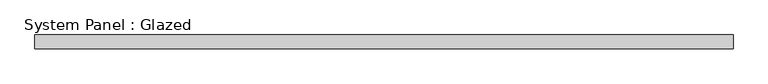
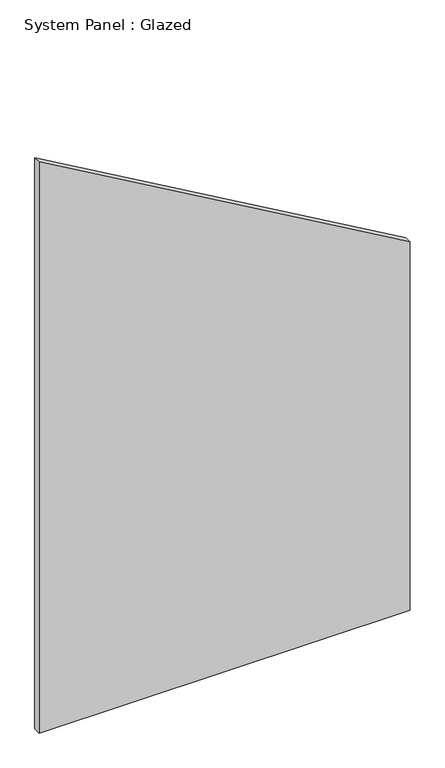
"""IFC4 building model written with IfcOpenShell, lengths in millimetres: plate geometry, System Panel : Glazed."""

from ifc_helpers import new_model, si_unit, frame, origin, place, context, project, spatial, polyline, outline, extrude, source, transform, mapped, element, save


def system_panel_glazed_d27e4e3c(model_context):
    return source(origin(), model_context, "Body", "SweptSolid", [
        extrude(outline(polyline([(0.0, -639.2857142), (0.0, 639.2857142), (1342.1254748, 639.2857142), (2080.3090332, -639.2857142), (0.0, -639.2857142)])), frame((0.0, 24.5, 0.0), z_axis=(0.0, 1.0, 0.0), x_axis=(0.0, 0.0, 1.0)), (0.0, 0.0, 1.0), 25.0),
    ])


if __name__ == "__main__":
    model = new_model("IFC4")
    model_context = context("Model", 3, world=origin())
    ifc_project = project(units=[si_unit("LENGTHUNIT", "METRE", prefix="MILLI")], contexts=[model_context])
    site = spatial("IfcSite", under=ifc_project)
    building = spatial("IfcBuilding", under=site)
    placement = place(None, origin())
    system_panel_glazed_shape = system_panel_glazed_d27e4e3c(model_context)
    element("IfcPlate", 1, ObjectType="System Panel : Glazed", at=placement, inside=building, context=model_context, shape_type="MappedRepresentation", body=[
        mapped(system_panel_glazed_shape, transform((0.0, 0.0, 0.0), x_axis=(1.0, 0.0, 0.0), y_axis=(0.0, 1.0, 0.0), z_axis=(0.0, 0.0, 1.0))),
    ])
    save(model, "model.ifc")

# Revit data of these elements
# Type "System Panel : Glazed"
#   Construction Type Id = "GSP4R"
#   Analytic Construction = "1/8 in Pilkington single glazing"
#   Visual Light Transmittance = 0.9
#   Solar Heat Gain Coefficient = 0.86
#   Heat Transfer Coefficient (U) = 6.7069 W/(m²·K)
#   Define Thermal Properties by = 1
# Element 1 (IfcPlate, "System Panel : Glazed")
#   Materials on its faces: "Glass"
# Materials
#   "Glass": class "Glass", colour RGB 0 128 192, transparency 0.75, Description = "Soda Lime Glass", Cost = 0
